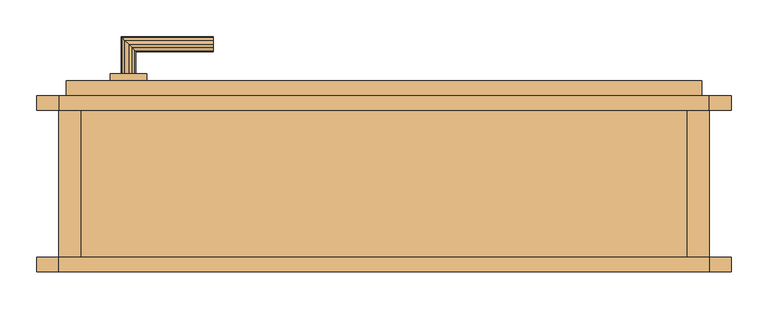
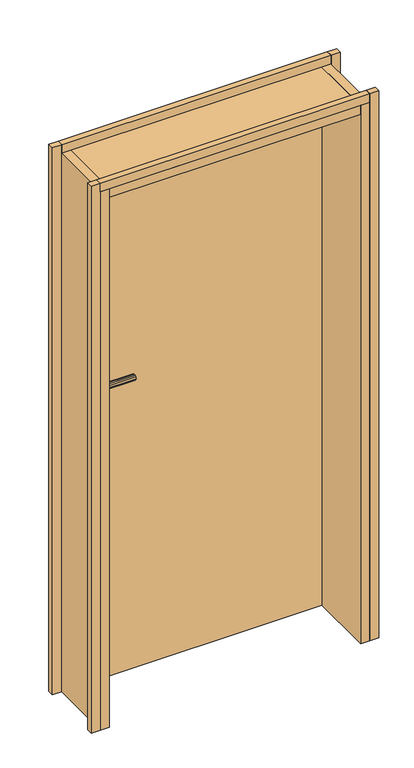
"""IFC4 building model written with IfcOpenShell, lengths in millimetres: door geometry, Tür."""

from ifc_helpers import new_model, si_unit, frame, origin, place, context, project, spatial, polyline, outline, extrude, faceted_brep, source, transform, mapped, element, save


def door_c6220e3f(model_context):
    return source(origin(), model_context, "Body", "SolidModel", [
        extrude(outline(polyline([(885.0, -20.0), (0.0, -20.0), (0.0, 0.0), (885.0, 0.0), (885.0, -20.0)])), frame((0.0, 0.0, 2010.0), z_axis=(0.0, 0.0, 1.0), x_axis=(1.0, 0.0, 0.0)), (0.0, 0.0, 1.0), 30.0),
        extrude(outline(polyline([(0.0, -20.0), (-30.0, -20.0), (-30.0, 0.0), (0.0, 0.0), (0.0, -20.0)])), frame((0.0, 0.0, 140.0), z_axis=(0.0, 0.0, 1.0), x_axis=(1.0, 0.0, 0.0)), (0.0, 0.0, 1.0), 1900.0),
        extrude(outline(polyline([(885.0, -20.0), (855.0, -20.0), (855.0, 220.0), (885.0, 220.0), (885.0, -20.0)])), frame((0.0, 0.0, 140.0), z_axis=(0.0, 0.0, 1.0), x_axis=(1.0, 0.0, 0.0)), (0.0, 0.0, 1.0), 1870.0),
        extrude(outline(polyline([(70.0, 190.0), (70.0, 200.0), (120.0, 200.0), (120.0, 190.0), (70.0, 190.0)])), frame((0.0, 0.0, 1050.0), z_axis=(0.0, 0.0, 1.0), x_axis=(1.0, 0.0, 0.0)), (0.0, 0.0, 1.0), 215.0),
        faceted_brep([(90.0, 190.0, 1198.660254), (95.0, 190.0, 1200.0), (100.0, 190.0, 1198.660254), (103.660254, 190.0, 1195.0), (105.0, 190.0, 1190.0), (103.660254, 190.0, 1185.0), (100.0, 190.0, 1181.339746), (95.0, 190.0, 1180.0), (90.0, 190.0, 1181.339746), (86.339746, 190.0, 1185.0), (85.0, 190.0, 1190.0), (86.339746, 190.0, 1195.0), (95.0, 150.0, 1200.0), (90.0, 145.0, 1198.660254), (86.339746, 141.339746, 1195.0), (85.0, 140.0, 1190.0), (86.339746, 141.339746, 1185.0), (90.0, 145.0, 1181.339746), (95.0, 150.0, 1180.0), (100.0, 155.0, 1181.339746), (103.660254, 158.660254, 1185.0), (105.0, 160.0, 1190.0), (103.660254, 158.660254, 1195.0), (100.0, 155.0, 1198.660254), (210.0, 155.0, 1198.660254), (210.0, 150.0, 1200.0), (210.0, 145.0, 1198.660254), (210.0, 141.339746, 1195.0), (210.0, 140.0, 1190.0), (210.0, 141.339746, 1185.0), (210.0, 145.0, 1181.339746), (210.0, 150.0, 1180.0), (210.0, 155.0, 1181.339746), (210.0, 158.660254, 1185.0), (210.0, 160.0, 1190.0), (210.0, 158.660254, 1195.0)], [[[0, 1, 2, 3, 4, 5, 6, 7, 8, 9, 10, 11]], [[12, 1, 0, 13]], [[13, 0, 11, 14]], [[14, 11, 10, 15]], [[15, 10, 9, 16]], [[16, 9, 8, 17]], [[17, 8, 7, 18]], [[18, 7, 6, 19]], [[19, 6, 5, 20]], [[20, 5, 4, 21]], [[21, 4, 3, 22]], [[22, 3, 2, 23]], [[23, 2, 1, 12]], [[24, 25, 26, 27, 28, 29, 30, 31, 32, 33, 34, 35]], [[25, 12, 13, 26]], [[26, 13, 14, 27]], [[27, 14, 15, 28]], [[28, 15, 16, 29]], [[29, 16, 17, 30]], [[30, 17, 18, 31]], [[31, 18, 19, 32]], [[32, 19, 20, 33]], [[33, 20, 21, 34]], [[34, 21, 22, 35]], [[35, 22, 23, 24]], [[24, 23, 12, 25]]]),
        faceted_brep([(100.0, 250.0, 1198.660254), (95.0, 250.0, 1200.0), (90.0, 250.0, 1198.660254), (86.339746, 250.0, 1195.0), (85.0, 250.0, 1190.0), (86.339746, 250.0, 1185.0), (90.0, 250.0, 1181.339746), (95.0, 250.0, 1180.0), (100.0, 250.0, 1181.339746), (103.660254, 250.0, 1185.0), (105.0, 250.0, 1190.0), (103.660254, 250.0, 1195.0), (95.0, 290.0, 1200.0), (90.0, 295.0, 1198.660254), (86.339746, 298.660254, 1195.0), (85.0, 300.0, 1190.0), (86.339746, 298.660254, 1185.0), (90.0, 295.0, 1181.339746), (95.0, 290.0, 1180.0), (100.0, 285.0, 1181.339746), (103.660254, 281.339746, 1185.0), (105.0, 280.0, 1190.0), (103.660254, 281.339746, 1195.0), (100.0, 285.0, 1198.660254), (210.0, 295.0, 1198.660254), (210.0, 290.0, 1200.0), (210.0, 285.0, 1198.660254), (210.0, 281.339746, 1195.0), (210.0, 280.0, 1190.0), (210.0, 281.339746, 1185.0), (210.0, 285.0, 1181.339746), (210.0, 290.0, 1180.0), (210.0, 295.0, 1181.339746), (210.0, 298.660254, 1185.0), (210.0, 300.0, 1190.0), (210.0, 298.660254, 1195.0)], [[[0, 1, 2, 3, 4, 5, 6, 7, 8, 9, 10, 11]], [[2, 1, 12, 13]], [[3, 2, 13, 14]], [[4, 3, 14, 15]], [[5, 4, 15, 16]], [[6, 5, 16, 17]], [[7, 6, 17, 18]], [[8, 7, 18, 19]], [[9, 8, 19, 20]], [[10, 9, 20, 21]], [[11, 10, 21, 22]], [[0, 11, 22, 23]], [[1, 0, 23, 12]], [[24, 25, 26, 27, 28, 29, 30, 31, 32, 33, 34, 35]], [[13, 12, 25, 24]], [[14, 13, 24, 35]], [[15, 14, 35, 34]], [[16, 15, 34, 33]], [[17, 16, 33, 32]], [[18, 17, 32, 31]], [[19, 18, 31, 30]], [[20, 19, 30, 29]], [[21, 20, 29, 28]], [[22, 21, 28, 27]], [[23, 22, 27, 26]], [[12, 23, 26, 25]]]),
        extrude(outline(polyline([(0.0, 200.0), (-30.0, 200.0), (-30.0, 220.0), (0.0, 220.0), (0.0, 200.0)])), frame((0.0, 0.0, 140.0), z_axis=(0.0, 0.0, 1.0), x_axis=(1.0, 0.0, 0.0)), (0.0, 0.0, 1.0), 1900.0),
        extrude(outline(polyline([(120.0, 240.0), (70.0, 240.0), (70.0, 250.0), (120.0, 250.0), (120.0, 240.0)])), frame((0.0, 0.0, 1050.0), z_axis=(0.0, 0.0, 1.0), x_axis=(1.0, 0.0, 0.0)), (0.0, 0.0, 1.0), 215.0),
        extrude(outline(polyline([(30.0, -20.0), (0.0, -20.0), (0.0, 220.0), (30.0, 220.0), (30.0, -20.0)])), frame((0.0, 0.0, 140.0), z_axis=(0.0, 0.0, 1.0), x_axis=(1.0, 0.0, 0.0)), (0.0, 0.0, 1.0), 1870.0),
        extrude(outline(polyline([(915.0, 220.0), (915.0, 200.0), (885.0, 200.0), (885.0, 220.0), (915.0, 220.0)])), frame((0.0, 0.0, 140.0), z_axis=(0.0, 0.0, 1.0), x_axis=(1.0, 0.0, 0.0)), (0.0, 0.0, 1.0), 1900.0),
        extrude(outline(polyline([(915.0, 0.0), (915.0, -20.0), (885.0, -20.0), (885.0, 0.0), (915.0, 0.0)])), frame((0.0, 0.0, 140.0), z_axis=(0.0, 0.0, 1.0), x_axis=(1.0, 0.0, 0.0)), (0.0, 0.0, 1.0), 1900.0),
        extrude(outline(polyline([(855.0, -20.0), (30.0, -20.0), (30.0, 220.0), (855.0, 220.0), (855.0, -20.0)])), frame((0.0, 0.0, 1980.0), z_axis=(0.0, 0.0, 1.0), x_axis=(1.0, 0.0, 0.0)), (0.0, 0.0, 1.0), 30.0),
        extrude(outline(polyline([(885.0, 200.0), (0.0, 200.0), (0.0, 220.0), (885.0, 220.0), (885.0, 200.0)])), frame((0.0, 0.0, 2010.0), z_axis=(0.0, 0.0, 1.0), x_axis=(1.0, 0.0, 0.0)), (0.0, 0.0, 1.0), 30.0),
        extrude(outline(polyline([(875.0, 200.0), (10.0, 200.0), (10.0, 240.0), (875.0, 240.0), (875.0, 200.0)])), frame((0.0, 0.0, 140.0), z_axis=(0.0, 0.0, 1.0), x_axis=(1.0, 0.0, 0.0)), (0.0, 0.0, 1.0), 1860.0),
    ])


if __name__ == "__main__":
    model = new_model("IFC4")
    model_context = context("Model", 3, world=origin())
    ifc_project = project(units=[si_unit("LENGTHUNIT", "METRE", prefix="MILLI")], contexts=[model_context])
    site = spatial("IfcSite", under=ifc_project)
    building = spatial("IfcBuilding", under=site)
    placement = place(None, origin())
    door_shape = door_c6220e3f(model_context)
    element("IfcDoor", 1, ObjectType="Tür", at=placement, inside=building, context=model_context, shape_type="MappedRepresentation", body=[
        mapped(door_shape, transform((0.0, 0.0, 0.0), x_axis=(1.0, 0.0, 0.0), y_axis=(0.0, 1.0, 0.0), z_axis=(0.0, 0.0, 1.0))),
    ])
    save(model, "model.ifc")

# Revit data of these elements
# Type "Tür"
#   Type Mark = "32"
# Element 1 (IfcDoor, "Tür")
#   Materials on its faces: "tuer_beschlag", "tuer_holzzarge"
# Materials
#   "tuer_beschlag": class "Unassigned", colour RGB 128 128 128, transparency 0
#   "tuer_holzzarge": class "Unassigned", colour RGB 255 255 255, transparency 0
